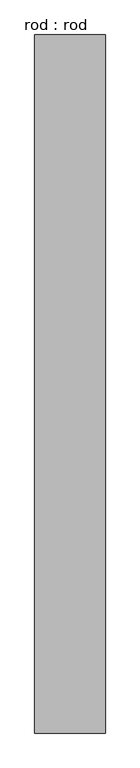
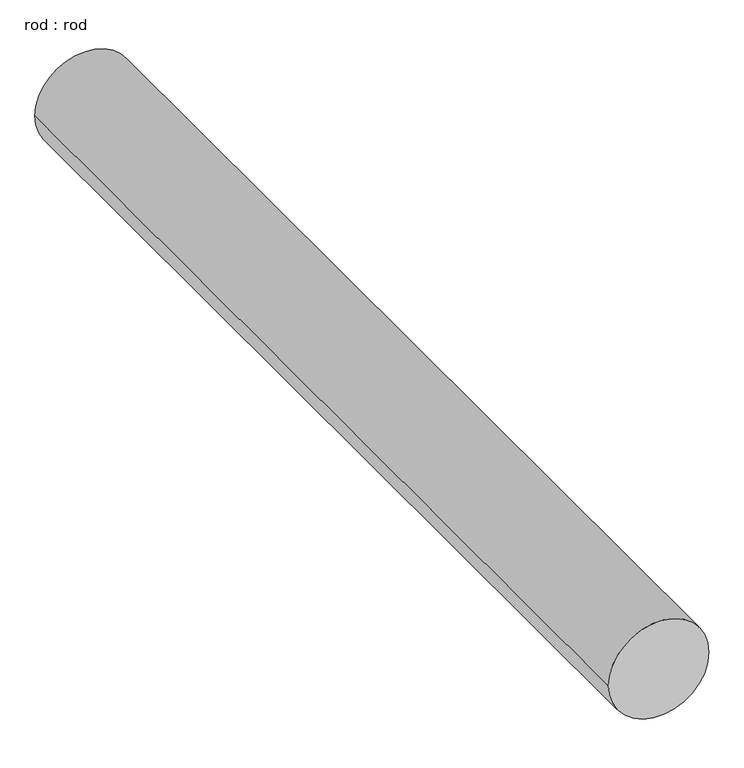
"""IFC4 building model written with IfcOpenShell, lengths in millimetres: proxy geometry, rod : rod."""

from ifc_helpers import new_model, si_unit, point, frame, frame_2d, origin, place, context, project, spatial, circle_curve, trimmed, segment, composite_curve, outline, extrude, source, transform, mapped, element, save


def rod_rod_db997cec(model_context):
    return source(origin(), model_context, "Body", "SweptSolid", [
        extrude(outline(composite_curve([segment(trimmed(circle_curve(frame_2d((0.0108462, 0.0)), 200.0), [point((0.0108462, 200.0))], [point((0.0108462, -200.0))], False, "CARTESIAN"), True, "CONTINUOUS"), segment(trimmed(circle_curve(frame_2d((0.0108462, 0.0)), 200.0), [point((0.0108462, -200.0))], [point((0.0108462, 200.0))], False, "CARTESIAN"), True, "CONTINUOUS")], self_intersect=False)), frame((0.0, 2116.7336128, 0.0), z_axis=(0.0, 1.0, 0.0), x_axis=(0.0, 0.0, 1.0)), (0.0, 0.0, 1.0), 3951.990005),
    ])


if __name__ == "__main__":
    model = new_model("IFC4")
    model_context = context("Model", 3, world=origin())
    ifc_project = project(units=[si_unit("LENGTHUNIT", "METRE", prefix="MILLI")], contexts=[model_context])
    site = spatial("IfcSite", under=ifc_project)
    building = spatial("IfcBuilding", under=site)
    placement = place(None, origin())
    rod_rod_shape = rod_rod_db997cec(model_context)
    element("IfcBuildingElementProxy", 1, Name="rod : rod", ObjectType="rod : rod", at=placement, inside=building, context=model_context, shape_type="MappedRepresentation", body=[
        mapped(rod_rod_shape, transform((0.0, 0.0, 0.0), x_axis=(1.0, 0.0, 0.0), y_axis=(0.0, 1.0, 0.0), z_axis=(0.0, 0.0, 1.0))),
    ])
    save(model, "model.ifc")

# Revit data of these elements
# Type "rod : rod"
#   Default Elevation = 0
